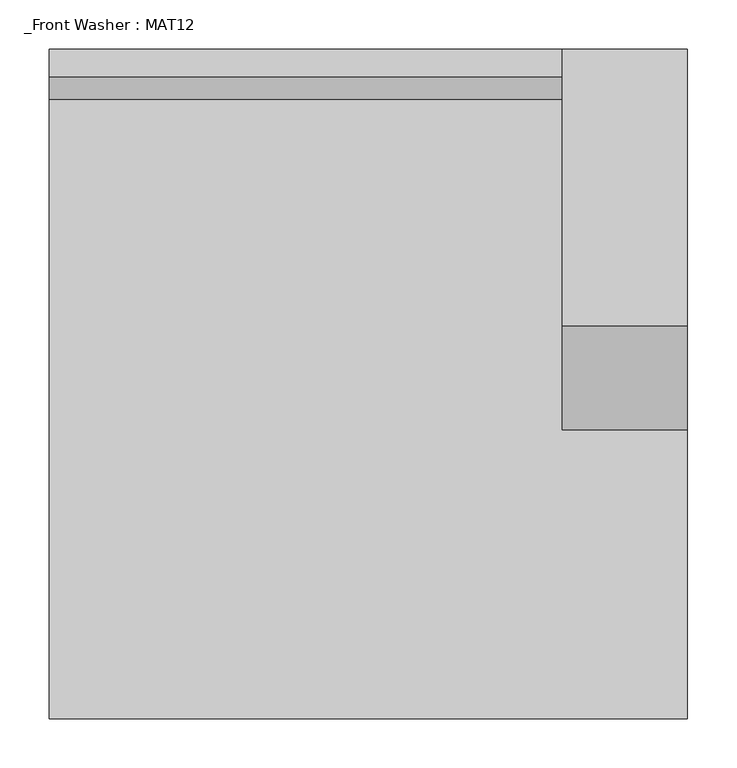
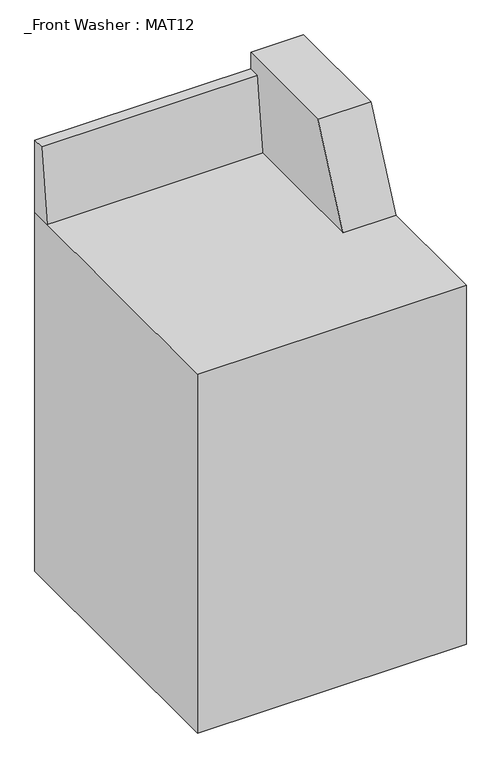
"""IFC4 building model written with IfcOpenShell, lengths in millimetres: proxy geometry, _Front Washer : MAT12."""

from ifc_helpers import new_model, si_unit, origin, origin_with_axes, place, context, project, spatial, polyline, outline, extrude, faceted_brep, source, transform, mapped, element, save


def front_washer_mat12_c85a6320(model_context):
    return source(origin(), model_context, "Body", "SolidModel", [
        faceted_brep([(434.6013644, 679.45, 914.4), (434.6013644, 679.45, 1139.825), (434.6013644, 398.5694732, 1139.825), (434.6013644, 293.4520693, 914.4), (307.6013644, 293.4520693, 914.4), (307.6013644, 398.5694732, 1139.825), (307.6013644, 679.45, 1139.825), (307.6013644, 679.45, 1098.55), (307.6013644, 651.66875, 1098.55), (307.6013644, 628.65, 914.4), (-213.0986356, 628.65, 914.4), (-213.0986356, 679.45, 914.4), (-213.0986356, 679.45, 1098.55), (-213.0986356, 651.66875, 1098.55)], [[[0, 1, 2, 3]], [[4, 5, 6, 7, 8, 9]], [[2, 1, 6, 5]], [[3, 2, 5, 4]], [[3, 4, 9, 10, 11, 0]], [[6, 1, 0, 11, 12, 7]], [[12, 11, 10, 13]], [[12, 13, 8, 7]], [[13, 10, 9, 8]]]),
        extrude(outline(polyline([(434.6013644, 0.0), (-213.0986356, 0.0), (-213.0986356, 679.45), (434.6013644, 679.45), (434.6013644, 0.0)])), origin_with_axes(), (0.0, 0.0, 1.0), 914.4),
    ])


if __name__ == "__main__":
    model = new_model("IFC4")
    model_context = context("Model", 3, world=origin())
    ifc_project = project(units=[si_unit("LENGTHUNIT", "METRE", prefix="MILLI")], contexts=[model_context])
    site = spatial("IfcSite", under=ifc_project)
    building = spatial("IfcBuilding", under=site)
    placement = place(None, origin())
    front_washer_mat12_shape = front_washer_mat12_c85a6320(model_context)
    element("IfcBuildingElementProxy", 1, Name="_Front Washer : MAT12", ObjectType="_Front Washer : MAT12", at=placement, inside=building, context=model_context, shape_type="MappedRepresentation", body=[
        mapped(front_washer_mat12_shape, transform((0.0, 0.0, 0.0), x_axis=(1.0, 0.0, 0.0), y_axis=(0.0, 1.0, 0.0), z_axis=(0.0, 0.0, 1.0))),
    ])
    save(model, "model.ifc")

# Revit data of these elements
# Type "_Front Washer : MAT12"
#   Type Mark = "MAT12"
#   Water_Pressure = "0"
#   Water_Flow_Rate = "0"
#   URL = "http://www.continentalgirbau.com"
#   Test Data = ""
#   Specification = "http://www.arcat.com/sd/clients/cogirbau.html?coid=44467"
#   SpecWizard = "http://www.arcat.com/specwizard/11110con/index.htm?mf=&coid=44467"
#   Send Message = "http://admin.arcat.com/users.pl?action=UserEmail&company=Continental%20Girbau,%20Inc.&coid=44467&rep=132&fax=920-231-4666 &mf="
#   Sales Information = ""
#   Product Properties = "http://www.arcat.com/bim/bim_info.pl?fn=Commercial_Washer"
#   Product Data = "http://www.arcat.com/arcatcos/cos44/arc44467.html"
#   Perf_WashSpeed = "44/67 rpm"
#   Perf_SpinSpeed = "710/473 rpm"
#   Perf_G-Force = "2.3/93 G"
#   Model = "H-Series"
#   Mech_Steam-Pressure = "29-87 psi"
#   Mech_Steam-Flow = "0"
#   Manufacturer Website = "http://www.continentalgirbau.com"
#   Manufacturer Phone - Toll Free = "800-256-1073 "
#   Manufacturer Phone = "920-231-8222 "
#   Manufacturer Fax = "920-231-4666 "
#   Manufacturer Address = "2500 State Rd. 44; Oshkosh; WI 54904\r\n"
#   Manufacturer = "Continental Girbau, Inc.\r\n"
#   Keynote = "11 23 00"
#   Installation-Fabrication = ""
#   Installation Phase = "Interior Fittings"
#   Green Building-LEED = "http://www.arcat.com/green/clients/leed_data_44467.html"
#   Drawn By = "Robert S. Weygant, CSI, CDT, SCIP"
#   Description = "Commercial Washer"
#   Copyright = "2009, ARCAT, Inc."
#   Construction Details = "http://www.arcat.com/details/cogirbau/cogirbau.html?coid=44467"
#   Compressed_Air_Pressure = "0"
#   Compressed_Air_Flow = "0"
#   Building Codes = ""
#   Assembly Code = "E1010610"
#   Three Phase = 0 VA
#   Single Phase = 0 VA
#   VOLTAGE = 240 V
#   OpeningCL = 0' - 7 7/8"
#   Mech_steam = 0' - 0 1/2"
#   Mech_HW = 0' - 0 3/8"
#   Mech_CW = 0' - 0 3/8"
#   MechWaste = 0' - 0 3/8"
#   MachWidth = 2' - 1 1/2"
#   MachHeight = 3' - 0"
#   MachDepth = 2' - 2 3/4"
#   LwrPanHt = 1' - 0"
#   InstWidth = 1' - 7 69/256"
#   Height of Back Panel = 3' - 7 1/4"
#   Height at Coin Insert = 3' - 8 7/8"
#   GlassCL = 0' - 5 7/8"
#   Fr_FaceWdth = 0' - 4 1/4"
#   DoorOpening = 1' - 3 3/4"
#   DoorHeight = 1' - 6"
#   Cyl_Diam = 1' - 0"
#   Cyl_Depth = 1' - 9"
#   CylRad = 0' - 6"
#   Compressed_Air_Connection = 0' - 2"
#   Capacity_Weight = 55
#   Capacity_Volume = 1.37445 (stored number, unit not read)
#   Warranty Duration (Years) = 0
#   Maintenance Schedule (Months) = 0
#   Expected Lifespan (Years) = 0
#   Trim Material = Painted Metal - Black
#   Shell Material = Stainless Steel
# Element 1 (IfcBuildingElementProxy, "_Front Washer : MAT12")
#   Materials on its faces: "Stainless Steel"
# Materials
#   "Painted Metal - Black": class "Unassigned", colour RGB 223 223 223, transparency 0, Cost = 0
#   "Stainless Steel": class "Unassigned", colour RGB 247 247 247, transparency 0
